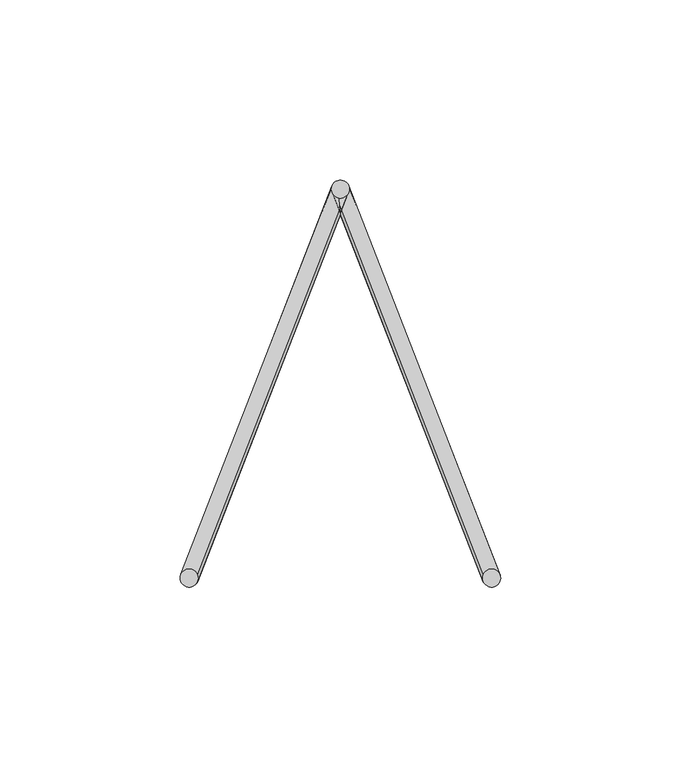
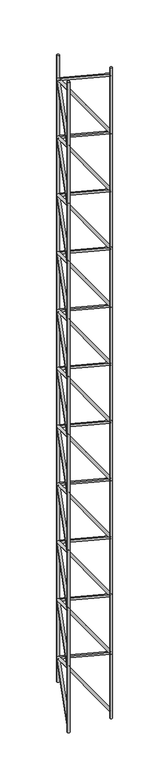
"""IFC4 building model written with IfcOpenShell, lengths in millimetres: proxy geometry, Pre-fab. (Vigota 1 - Pano 21)."""

from ifc_helpers import new_model, si_unit, point, frame, frame_2d, origin, origin_with_axes, origin_2d, place, context, project, spatial, circle_curve, trimmed, segment, composite_curve, outline, extrude, source, transform, mapped, element, save


def structural_framing_493db843(model_context):
    return source(origin(), model_context, "Body", "SweptSolid", [
        extrude(outline(composite_curve([segment(trimmed(circle_curve(origin_2d(), 2.5), [point((2.5, 0.0))], [point((-2.5, 0.0))], False, "CARTESIAN"), True, "CONTINUOUS"), segment(trimmed(circle_curve(origin_2d(), 2.5), [point((-2.5, 0.0))], [point((2.5, 0.0))], False, "CARTESIAN"), True, "CONTINUOUS")], self_intersect=False)), origin_with_axes(), (0.0, 0.0, 1.0), 1348.99893),
        extrude(outline(composite_curve([segment(trimmed(circle_curve(frame_2d((-42.0, 108.0)), 2.5), [point((-39.5, 108.0))], [point((-44.5, 108.0))], False, "CARTESIAN"), True, "CONTINUOUS"), segment(trimmed(circle_curve(frame_2d((-42.0, 108.0)), 2.5), [point((-44.5, 108.0))], [point((-39.5, 108.0))], False, "CARTESIAN"), True, "CONTINUOUS")], self_intersect=False)), frame((0.0, 0.0, 24.499465), z_axis=(0.0, 0.0, 1.0), x_axis=(1.0, 0.0, 0.0)), (0.0, 0.0, 1.0), 1300.0),
        extrude(outline(composite_curve([segment(trimmed(circle_curve(origin_2d(), 2.5), [point((2.5, 0.0))], [point((-2.5, 0.0))], False, "CARTESIAN"), True, "CONTINUOUS"), segment(trimmed(circle_curve(origin_2d(), 2.5), [point((-2.5, 0.0))], [point((2.5, 0.0))], False, "CARTESIAN"), True, "CONTINUOUS")], self_intersect=False)), frame((0.0, 0.0, 14.499465), z_axis=(-0.3218603428886276, 0.8276408817707567, 0.4598004898837537), x_axis=(0.8192319205108605, -3.936835275445103e-11, 0.5734623443750141)), (0.0, 0.0, 1.0), 130.491379),
        extrude(outline(composite_curve([segment(trimmed(circle_curve(origin_2d(), 2.5), [point((2.5, 0.0))], [point((-2.5, 0.0))], False, "CARTESIAN"), True, "CONTINUOUS"), segment(trimmed(circle_curve(origin_2d(), 2.5), [point((-2.5, 0.0))], [point((2.5, 0.0))], False, "CARTESIAN"), True, "CONTINUOUS")], self_intersect=False)), frame((-42.0, 108.0, 74.499465), z_axis=(0.3218603428886276, -0.8276408817707567, 0.4598004898837537), x_axis=(0.8192319205108605, -3.936835275445103e-11, -0.5734623443750141)), (0.0, 0.0, 1.0), 130.491379),
        extrude(outline(composite_curve([segment(trimmed(circle_curve(origin_2d(), 2.5), [point((2.5, 0.0))], [point((-2.5, 0.0))], False, "CARTESIAN"), True, "CONTINUOUS"), segment(trimmed(circle_curve(origin_2d(), 2.5), [point((-2.5, 0.0))], [point((2.5, 0.0))], False, "CARTESIAN"), True, "CONTINUOUS")], self_intersect=False)), frame((0.0, 0.0, 134.499465), z_axis=(-0.3218603428886276, 0.8276408817707567, 0.4598004898837537), x_axis=(0.8192319205108605, -3.936835275445103e-11, 0.5734623443750141)), (0.0, 0.0, 1.0), 130.491379),
        extrude(outline(composite_curve([segment(trimmed(circle_curve(origin_2d(), 2.5), [point((2.5, 0.0))], [point((-2.5, 0.0))], False, "CARTESIAN"), True, "CONTINUOUS"), segment(trimmed(circle_curve(origin_2d(), 2.5), [point((-2.5, 0.0))], [point((2.5, 0.0))], False, "CARTESIAN"), True, "CONTINUOUS")], self_intersect=False)), frame((-42.0, 108.0, 194.499465), z_axis=(0.3218603428886276, -0.8276408817707567, 0.4598004898837537), x_axis=(0.8192319205108605, -3.936835275445103e-11, -0.5734623443750141)), (0.0, 0.0, 1.0), 130.491379),
        extrude(outline(composite_curve([segment(trimmed(circle_curve(origin_2d(), 2.5), [point((2.5, 0.0))], [point((-2.5, 0.0))], False, "CARTESIAN"), True, "CONTINUOUS"), segment(trimmed(circle_curve(origin_2d(), 2.5), [point((-2.5, 0.0))], [point((2.5, 0.0))], False, "CARTESIAN"), True, "CONTINUOUS")], self_intersect=False)), frame((0.0, 0.0, 254.499465), z_axis=(-0.3218603428886276, 0.8276408817707567, 0.4598004898837537), x_axis=(0.8192319205108605, -3.936835275445103e-11, 0.5734623443750141)), (0.0, 0.0, 1.0), 130.491379),
        extrude(outline(composite_curve([segment(trimmed(circle_curve(origin_2d(), 2.5), [point((2.5, 0.0))], [point((-2.5, 0.0))], False, "CARTESIAN"), True, "CONTINUOUS"), segment(trimmed(circle_curve(origin_2d(), 2.5), [point((-2.5, 0.0))], [point((2.5, 0.0))], False, "CARTESIAN"), True, "CONTINUOUS")], self_intersect=False)), frame((-42.0, 108.0, 314.499465), z_axis=(0.3218603428886276, -0.8276408817707567, 0.4598004898837537), x_axis=(0.8192319205108605, -3.936835275445103e-11, -0.5734623443750141)), (0.0, 0.0, 1.0), 130.491379),
        extrude(outline(composite_curve([segment(trimmed(circle_curve(origin_2d(), 2.5), [point((2.5, 0.0))], [point((-2.5, 0.0))], False, "CARTESIAN"), True, "CONTINUOUS"), segment(trimmed(circle_curve(origin_2d(), 2.5), [point((-2.5, 0.0))], [point((2.5, 0.0))], False, "CARTESIAN"), True, "CONTINUOUS")], self_intersect=False)), frame((0.0, 0.0, 374.499465), z_axis=(-0.3218603428886276, 0.8276408817707567, 0.4598004898837537), x_axis=(0.8192319205108605, -3.936835275445103e-11, 0.5734623443750141)), (0.0, 0.0, 1.0), 130.491379),
        extrude(outline(composite_curve([segment(trimmed(circle_curve(origin_2d(), 2.5), [point((2.5, 0.0))], [point((-2.5, 0.0))], False, "CARTESIAN"), True, "CONTINUOUS"), segment(trimmed(circle_curve(origin_2d(), 2.5), [point((-2.5, 0.0))], [point((2.5, 0.0))], False, "CARTESIAN"), True, "CONTINUOUS")], self_intersect=False)), frame((-42.0, 108.0, 434.499465), z_axis=(0.3218603428886276, -0.8276408817707567, 0.4598004898837537), x_axis=(0.8192319205108605, -3.936835275445103e-11, -0.5734623443750141)), (0.0, 0.0, 1.0), 130.491379),
        extrude(outline(composite_curve([segment(trimmed(circle_curve(origin_2d(), 2.5), [point((2.5, 0.0))], [point((-2.5, 0.0))], False, "CARTESIAN"), True, "CONTINUOUS"), segment(trimmed(circle_curve(origin_2d(), 2.5), [point((-2.5, 0.0))], [point((2.5, 0.0))], False, "CARTESIAN"), True, "CONTINUOUS")], self_intersect=False)), frame((0.0, 0.0, 494.499465), z_axis=(-0.3218603428886276, 0.8276408817707567, 0.4598004898837537), x_axis=(0.8192319205108605, -3.936835275445103e-11, 0.5734623443750141)), (0.0, 0.0, 1.0), 130.491379),
        extrude(outline(composite_curve([segment(trimmed(circle_curve(origin_2d(), 2.5), [point((2.5, 0.0))], [point((-2.5, 0.0))], False, "CARTESIAN"), True, "CONTINUOUS"), segment(trimmed(circle_curve(origin_2d(), 2.5), [point((-2.5, 0.0))], [point((2.5, 0.0))], False, "CARTESIAN"), True, "CONTINUOUS")], self_intersect=False)), frame((-42.0, 108.0, 554.499465), z_axis=(0.3218603428886276, -0.8276408817707567, 0.4598004898837537), x_axis=(0.8192319205108605, -3.936835275445103e-11, -0.5734623443750141)), (0.0, 0.0, 1.0), 130.491379),
        extrude(outline(composite_curve([segment(trimmed(circle_curve(origin_2d(), 2.5), [point((2.5, 0.0))], [point((-2.5, 0.0))], False, "CARTESIAN"), True, "CONTINUOUS"), segment(trimmed(circle_curve(origin_2d(), 2.5), [point((-2.5, 0.0))], [point((2.5, 0.0))], False, "CARTESIAN"), True, "CONTINUOUS")], self_intersect=False)), frame((0.0, 0.0, 614.499465), z_axis=(-0.3218603428886276, 0.8276408817707567, 0.4598004898837537), x_axis=(0.8192319205108605, -3.936835275445103e-11, 0.5734623443750141)), (0.0, 0.0, 1.0), 130.491379),
        extrude(outline(composite_curve([segment(trimmed(circle_curve(origin_2d(), 2.5), [point((2.5, 0.0))], [point((-2.5, 0.0))], False, "CARTESIAN"), True, "CONTINUOUS"), segment(trimmed(circle_curve(origin_2d(), 2.5), [point((-2.5, 0.0))], [point((2.5, 0.0))], False, "CARTESIAN"), True, "CONTINUOUS")], self_intersect=False)), frame((-42.0, 108.0, 674.499465), z_axis=(0.3218603428886276, -0.8276408817707567, 0.4598004898837537), x_axis=(0.8192319205108605, -3.936835275445103e-11, -0.5734623443750141)), (0.0, 0.0, 1.0), 130.491379),
        extrude(outline(composite_curve([segment(trimmed(circle_curve(origin_2d(), 2.5), [point((2.5, 0.0))], [point((-2.5, 0.0))], False, "CARTESIAN"), True, "CONTINUOUS"), segment(trimmed(circle_curve(origin_2d(), 2.5), [point((-2.5, 0.0))], [point((2.5, 0.0))], False, "CARTESIAN"), True, "CONTINUOUS")], self_intersect=False)), frame((0.0, 0.0, 734.499465), z_axis=(-0.3218603428886276, 0.8276408817707567, 0.4598004898837537), x_axis=(0.8192319205108605, -3.936835275445103e-11, 0.5734623443750141)), (0.0, 0.0, 1.0), 130.491379),
        extrude(outline(composite_curve([segment(trimmed(circle_curve(origin_2d(), 2.5), [point((2.5, 0.0))], [point((-2.5, 0.0))], False, "CARTESIAN"), True, "CONTINUOUS"), segment(trimmed(circle_curve(origin_2d(), 2.5), [point((-2.5, 0.0))], [point((2.5, 0.0))], False, "CARTESIAN"), True, "CONTINUOUS")], self_intersect=False)), frame((-42.0, 108.0, 794.499465), z_axis=(0.3218603428886276, -0.8276408817707567, 0.4598004898837537), x_axis=(0.8192319205108605, -3.936835275445103e-11, -0.5734623443750141)), (0.0, 0.0, 1.0), 130.491379),
        extrude(outline(composite_curve([segment(trimmed(circle_curve(origin_2d(), 2.5), [point((2.5, 0.0))], [point((-2.5, 0.0))], False, "CARTESIAN"), True, "CONTINUOUS"), segment(trimmed(circle_curve(origin_2d(), 2.5), [point((-2.5, 0.0))], [point((2.5, 0.0))], False, "CARTESIAN"), True, "CONTINUOUS")], self_intersect=False)), frame((0.0, 0.0, 854.499465), z_axis=(-0.3218603428886276, 0.8276408817707567, 0.4598004898837537), x_axis=(0.8192319205108605, -3.936835275445103e-11, 0.5734623443750141)), (0.0, 0.0, 1.0), 130.491379),
        extrude(outline(composite_curve([segment(trimmed(circle_curve(origin_2d(), 2.5), [point((2.5, 0.0))], [point((-2.5, 0.0))], False, "CARTESIAN"), True, "CONTINUOUS"), segment(trimmed(circle_curve(origin_2d(), 2.5), [point((-2.5, 0.0))], [point((2.5, 0.0))], False, "CARTESIAN"), True, "CONTINUOUS")], self_intersect=False)), frame((-42.0, 108.0, 914.499465), z_axis=(0.3218603428886276, -0.8276408817707567, 0.4598004898837537), x_axis=(0.8192319205108605, -3.936835275445103e-11, -0.5734623443750141)), (0.0, 0.0, 1.0), 130.491379),
        extrude(outline(composite_curve([segment(trimmed(circle_curve(origin_2d(), 2.5), [point((2.5, 0.0))], [point((-2.5, 0.0))], False, "CARTESIAN"), True, "CONTINUOUS"), segment(trimmed(circle_curve(origin_2d(), 2.5), [point((-2.5, 0.0))], [point((2.5, 0.0))], False, "CARTESIAN"), True, "CONTINUOUS")], self_intersect=False)), frame((0.0, 0.0, 974.499465), z_axis=(-0.3218603428886276, 0.8276408817707567, 0.4598004898837537), x_axis=(0.8192319205108605, -3.936835275445103e-11, 0.5734623443750141)), (0.0, 0.0, 1.0), 130.491379),
        extrude(outline(composite_curve([segment(trimmed(circle_curve(origin_2d(), 2.5), [point((2.5, 0.0))], [point((-2.5, 0.0))], False, "CARTESIAN"), True, "CONTINUOUS"), segment(trimmed(circle_curve(origin_2d(), 2.5), [point((-2.5, 0.0))], [point((2.5, 0.0))], False, "CARTESIAN"), True, "CONTINUOUS")], self_intersect=False)), frame((-42.0, 108.0, 1034.499465), z_axis=(0.3218603428886276, -0.8276408817707567, 0.4598004898837537), x_axis=(0.8192319205108605, -3.936835275445103e-11, -0.5734623443750141)), (0.0, 0.0, 1.0), 130.491379),
        extrude(outline(composite_curve([segment(trimmed(circle_curve(origin_2d(), 2.5), [point((2.5, 0.0))], [point((-2.5, 0.0))], False, "CARTESIAN"), True, "CONTINUOUS"), segment(trimmed(circle_curve(origin_2d(), 2.5), [point((-2.5, 0.0))], [point((2.5, 0.0))], False, "CARTESIAN"), True, "CONTINUOUS")], self_intersect=False)), frame((0.0, 0.0, 1094.499465), z_axis=(-0.3218603428886276, 0.8276408817707567, 0.4598004898837537), x_axis=(0.8192319205108605, -3.936835275445103e-11, 0.5734623443750141)), (0.0, 0.0, 1.0), 130.491379),
        extrude(outline(composite_curve([segment(trimmed(circle_curve(origin_2d(), 2.5), [point((2.5, 0.0))], [point((-2.5, 0.0))], False, "CARTESIAN"), True, "CONTINUOUS"), segment(trimmed(circle_curve(origin_2d(), 2.5), [point((-2.5, 0.0))], [point((2.5, 0.0))], False, "CARTESIAN"), True, "CONTINUOUS")], self_intersect=False)), frame((-42.0, 108.0, 1154.499465), z_axis=(0.3218603428886276, -0.8276408817707567, 0.4598004898837537), x_axis=(0.8192319205108605, -3.936835275445103e-11, -0.5734623443750141)), (0.0, 0.0, 1.0), 130.491379),
        extrude(outline(composite_curve([segment(trimmed(circle_curve(origin_2d(), 2.5), [point((2.5, 0.0))], [point((-2.5, 0.0))], False, "CARTESIAN"), True, "CONTINUOUS"), segment(trimmed(circle_curve(origin_2d(), 2.5), [point((-2.5, 0.0))], [point((2.5, 0.0))], False, "CARTESIAN"), True, "CONTINUOUS")], self_intersect=False)), frame((0.0, 0.0, 1214.499465), z_axis=(-0.3218603428886276, 0.8276408817707567, 0.4598004898837537), x_axis=(0.8192319205108605, -3.936835275445103e-11, 0.5734623443750141)), (0.0, 0.0, 1.0), 130.491379),
        extrude(outline(composite_curve([segment(trimmed(circle_curve(origin_2d(), 2.5), [point((2.5, 0.0))], [point((-2.5, 0.0))], False, "CARTESIAN"), True, "CONTINUOUS"), segment(trimmed(circle_curve(origin_2d(), 2.5), [point((-2.5, 0.0))], [point((2.5, 0.0))], False, "CARTESIAN"), True, "CONTINUOUS")], self_intersect=False)), frame((-42.0, 108.0, 1274.499465), z_axis=(0.3218603428886276, -0.8276408817707567, 0.4598004898837537), x_axis=(0.8192319205108605, -3.936835275445103e-11, -0.5734623443750141)), (0.0, 0.0, 1.0), 130.491379),
        extrude(outline(composite_curve([segment(trimmed(circle_curve(frame_2d((-84.0, 0.0)), 2.5), [point((-81.5, 0.0))], [point((-86.5, 0.0))], False, "CARTESIAN"), True, "CONTINUOUS"), segment(trimmed(circle_curve(frame_2d((-84.0, 0.0)), 2.5), [point((-86.5, 0.0))], [point((-81.5, 0.0))], False, "CARTESIAN"), True, "CONTINUOUS")], self_intersect=False)), origin_with_axes(), (0.0, 0.0, 1.0), 1348.99893),
        extrude(outline(composite_curve([segment(trimmed(circle_curve(origin_2d(), 2.5), [point((2.5, 0.0))], [point((-2.5, 0.0))], False, "CARTESIAN"), True, "CONTINUOUS"), segment(trimmed(circle_curve(origin_2d(), 2.5), [point((-2.5, 0.0))], [point((2.5, 0.0))], False, "CARTESIAN"), True, "CONTINUOUS")], self_intersect=False)), frame((-84.0, 0.0, 14.499465), z_axis=(0.3218603428886276, 0.8276408817707567, 0.4598004898837537), x_axis=(0.8192319205108605, 3.936835275445103e-11, -0.5734623443750141)), (0.0, 0.0, 1.0), 130.491379),
        extrude(outline(composite_curve([segment(trimmed(circle_curve(origin_2d(), 2.5), [point((2.5, 0.0))], [point((-2.5, 0.0))], False, "CARTESIAN"), True, "CONTINUOUS"), segment(trimmed(circle_curve(origin_2d(), 2.5), [point((-2.5, 0.0))], [point((2.5, 0.0))], False, "CARTESIAN"), True, "CONTINUOUS")], self_intersect=False)), frame((-42.0, 108.0, 74.499465), z_axis=(-0.3218603428886276, -0.8276408817707567, 0.4598004898837537), x_axis=(0.8192319205108605, 3.936835275445103e-11, 0.5734623443750141)), (0.0, 0.0, 1.0), 130.491379),
        extrude(outline(composite_curve([segment(trimmed(circle_curve(origin_2d(), 2.5), [point((2.5, 0.0))], [point((-2.5, 0.0))], False, "CARTESIAN"), True, "CONTINUOUS"), segment(trimmed(circle_curve(origin_2d(), 2.5), [point((-2.5, 0.0))], [point((2.5, 0.0))], False, "CARTESIAN"), True, "CONTINUOUS")], self_intersect=False)), frame((-84.0, 0.0, 134.499465), z_axis=(0.3218603428886276, 0.8276408817707567, 0.4598004898837537), x_axis=(0.8192319205108605, 3.936835275445103e-11, -0.5734623443750141)), (0.0, 0.0, 1.0), 130.491379),
        extrude(outline(composite_curve([segment(trimmed(circle_curve(origin_2d(), 2.5), [point((2.5, 0.0))], [point((-2.5, 0.0))], False, "CARTESIAN"), True, "CONTINUOUS"), segment(trimmed(circle_curve(origin_2d(), 2.5), [point((-2.5, 0.0))], [point((2.5, 0.0))], False, "CARTESIAN"), True, "CONTINUOUS")], self_intersect=False)), frame((-42.0, 108.0, 194.499465), z_axis=(-0.3218603428886276, -0.8276408817707567, 0.4598004898837537), x_axis=(0.8192319205108605, 3.936835275445103e-11, 0.5734623443750141)), (0.0, 0.0, 1.0), 130.491379),
        extrude(outline(composite_curve([segment(trimmed(circle_curve(origin_2d(), 2.5), [point((2.5, 0.0))], [point((-2.5, 0.0))], False, "CARTESIAN"), True, "CONTINUOUS"), segment(trimmed(circle_curve(origin_2d(), 2.5), [point((-2.5, 0.0))], [point((2.5, 0.0))], False, "CARTESIAN"), True, "CONTINUOUS")], self_intersect=False)), frame((-84.0, 0.0, 254.499465), z_axis=(0.3218603428886276, 0.8276408817707567, 0.4598004898837537), x_axis=(0.8192319205108605, 3.936835275445103e-11, -0.5734623443750141)), (0.0, 0.0, 1.0), 130.491379),
        extrude(outline(composite_curve([segment(trimmed(circle_curve(origin_2d(), 2.5), [point((2.5, 0.0))], [point((-2.5, 0.0))], False, "CARTESIAN"), True, "CONTINUOUS"), segment(trimmed(circle_curve(origin_2d(), 2.5), [point((-2.5, 0.0))], [point((2.5, 0.0))], False, "CARTESIAN"), True, "CONTINUOUS")], self_intersect=False)), frame((-42.0, 108.0, 314.499465), z_axis=(-0.3218603428886276, -0.8276408817707567, 0.4598004898837537), x_axis=(0.8192319205108605, 3.936835275445103e-11, 0.5734623443750141)), (0.0, 0.0, 1.0), 130.491379),
        extrude(outline(composite_curve([segment(trimmed(circle_curve(origin_2d(), 2.5), [point((2.5, 0.0))], [point((-2.5, 0.0))], False, "CARTESIAN"), True, "CONTINUOUS"), segment(trimmed(circle_curve(origin_2d(), 2.5), [point((-2.5, 0.0))], [point((2.5, 0.0))], False, "CARTESIAN"), True, "CONTINUOUS")], self_intersect=False)), frame((-84.0, 0.0, 374.499465), z_axis=(0.3218603428886276, 0.8276408817707567, 0.4598004898837537), x_axis=(0.8192319205108605, 3.936835275445103e-11, -0.5734623443750141)), (0.0, 0.0, 1.0), 130.491379),
        extrude(outline(composite_curve([segment(trimmed(circle_curve(origin_2d(), 2.5), [point((2.5, 0.0))], [point((-2.5, 0.0))], False, "CARTESIAN"), True, "CONTINUOUS"), segment(trimmed(circle_curve(origin_2d(), 2.5), [point((-2.5, 0.0))], [point((2.5, 0.0))], False, "CARTESIAN"), True, "CONTINUOUS")], self_intersect=False)), frame((-42.0, 108.0, 434.499465), z_axis=(-0.3218603428886276, -0.8276408817707567, 0.4598004898837537), x_axis=(0.8192319205108605, 3.936835275445103e-11, 0.5734623443750141)), (0.0, 0.0, 1.0), 130.491379),
        extrude(outline(composite_curve([segment(trimmed(circle_curve(origin_2d(), 2.5), [point((2.5, 0.0))], [point((-2.5, 0.0))], False, "CARTESIAN"), True, "CONTINUOUS"), segment(trimmed(circle_curve(origin_2d(), 2.5), [point((-2.5, 0.0))], [point((2.5, 0.0))], False, "CARTESIAN"), True, "CONTINUOUS")], self_intersect=False)), frame((-84.0, 0.0, 494.499465), z_axis=(0.3218603428886276, 0.8276408817707567, 0.4598004898837537), x_axis=(0.8192319205108605, 3.936835275445103e-11, -0.5734623443750141)), (0.0, 0.0, 1.0), 130.491379),
        extrude(outline(composite_curve([segment(trimmed(circle_curve(origin_2d(), 2.5), [point((2.5, 0.0))], [point((-2.5, 0.0))], False, "CARTESIAN"), True, "CONTINUOUS"), segment(trimmed(circle_curve(origin_2d(), 2.5), [point((-2.5, 0.0))], [point((2.5, 0.0))], False, "CARTESIAN"), True, "CONTINUOUS")], self_intersect=False)), frame((-42.0, 108.0, 554.499465), z_axis=(-0.3218603428886276, -0.8276408817707567, 0.4598004898837537), x_axis=(0.8192319205108605, 3.936835275445103e-11, 0.5734623443750141)), (0.0, 0.0, 1.0), 130.491379),
        extrude(outline(composite_curve([segment(trimmed(circle_curve(origin_2d(), 2.5), [point((2.5, 0.0))], [point((-2.5, 0.0))], False, "CARTESIAN"), True, "CONTINUOUS"), segment(trimmed(circle_curve(origin_2d(), 2.5), [point((-2.5, 0.0))], [point((2.5, 0.0))], False, "CARTESIAN"), True, "CONTINUOUS")], self_intersect=False)), frame((-84.0, 0.0, 614.499465), z_axis=(0.3218603428886276, 0.8276408817707567, 0.4598004898837537), x_axis=(0.8192319205108605, 3.936835275445103e-11, -0.5734623443750141)), (0.0, 0.0, 1.0), 130.491379),
        extrude(outline(composite_curve([segment(trimmed(circle_curve(origin_2d(), 2.5), [point((2.5, 0.0))], [point((-2.5, 0.0))], False, "CARTESIAN"), True, "CONTINUOUS"), segment(trimmed(circle_curve(origin_2d(), 2.5), [point((-2.5, 0.0))], [point((2.5, 0.0))], False, "CARTESIAN"), True, "CONTINUOUS")], self_intersect=False)), frame((-42.0, 108.0, 674.499465), z_axis=(-0.3218603428886276, -0.8276408817707567, 0.4598004898837537), x_axis=(0.8192319205108605, 3.936835275445103e-11, 0.5734623443750141)), (0.0, 0.0, 1.0), 130.491379),
        extrude(outline(composite_curve([segment(trimmed(circle_curve(origin_2d(), 2.5), [point((2.5, 0.0))], [point((-2.5, 0.0))], False, "CARTESIAN"), True, "CONTINUOUS"), segment(trimmed(circle_curve(origin_2d(), 2.5), [point((-2.5, 0.0))], [point((2.5, 0.0))], False, "CARTESIAN"), True, "CONTINUOUS")], self_intersect=False)), frame((-84.0, 0.0, 734.499465), z_axis=(0.3218603428886276, 0.8276408817707567, 0.4598004898837537), x_axis=(0.8192319205108605, 3.936835275445103e-11, -0.5734623443750141)), (0.0, 0.0, 1.0), 130.491379),
        extrude(outline(composite_curve([segment(trimmed(circle_curve(origin_2d(), 2.5), [point((2.5, 0.0))], [point((-2.5, 0.0))], False, "CARTESIAN"), True, "CONTINUOUS"), segment(trimmed(circle_curve(origin_2d(), 2.5), [point((-2.5, 0.0))], [point((2.5, 0.0))], False, "CARTESIAN"), True, "CONTINUOUS")], self_intersect=False)), frame((-42.0, 108.0, 794.499465), z_axis=(-0.3218603428886276, -0.8276408817707567, 0.4598004898837537), x_axis=(0.8192319205108605, 3.936835275445103e-11, 0.5734623443750141)), (0.0, 0.0, 1.0), 130.491379),
        extrude(outline(composite_curve([segment(trimmed(circle_curve(origin_2d(), 2.5), [point((2.5, 0.0))], [point((-2.5, 0.0))], False, "CARTESIAN"), True, "CONTINUOUS"), segment(trimmed(circle_curve(origin_2d(), 2.5), [point((-2.5, 0.0))], [point((2.5, 0.0))], False, "CARTESIAN"), True, "CONTINUOUS")], self_intersect=False)), frame((-84.0, 0.0, 854.499465), z_axis=(0.3218603428886276, 0.8276408817707567, 0.4598004898837537), x_axis=(0.8192319205108605, 3.936835275445103e-11, -0.5734623443750141)), (0.0, 0.0, 1.0), 130.491379),
        extrude(outline(composite_curve([segment(trimmed(circle_curve(origin_2d(), 2.5), [point((2.5, 0.0))], [point((-2.5, 0.0))], False, "CARTESIAN"), True, "CONTINUOUS"), segment(trimmed(circle_curve(origin_2d(), 2.5), [point((-2.5, 0.0))], [point((2.5, 0.0))], False, "CARTESIAN"), True, "CONTINUOUS")], self_intersect=False)), frame((-42.0, 108.0, 914.499465), z_axis=(-0.3218603428886276, -0.8276408817707567, 0.4598004898837537), x_axis=(0.8192319205108605, 3.936835275445103e-11, 0.5734623443750141)), (0.0, 0.0, 1.0), 130.491379),
        extrude(outline(composite_curve([segment(trimmed(circle_curve(origin_2d(), 2.5), [point((2.5, 0.0))], [point((-2.5, 0.0))], False, "CARTESIAN"), True, "CONTINUOUS"), segment(trimmed(circle_curve(origin_2d(), 2.5), [point((-2.5, 0.0))], [point((2.5, 0.0))], False, "CARTESIAN"), True, "CONTINUOUS")], self_intersect=False)), frame((-84.0, 0.0, 974.499465), z_axis=(0.3218603428886276, 0.8276408817707567, 0.4598004898837537), x_axis=(0.8192319205108605, 3.936835275445103e-11, -0.5734623443750141)), (0.0, 0.0, 1.0), 130.491379),
        extrude(outline(composite_curve([segment(trimmed(circle_curve(origin_2d(), 2.5), [point((2.5, 0.0))], [point((-2.5, 0.0))], False, "CARTESIAN"), True, "CONTINUOUS"), segment(trimmed(circle_curve(origin_2d(), 2.5), [point((-2.5, 0.0))], [point((2.5, 0.0))], False, "CARTESIAN"), True, "CONTINUOUS")], self_intersect=False)), frame((-42.0, 108.0, 1034.499465), z_axis=(-0.3218603428886276, -0.8276408817707567, 0.4598004898837537), x_axis=(0.8192319205108605, 3.936835275445103e-11, 0.5734623443750141)), (0.0, 0.0, 1.0), 130.491379),
        extrude(outline(composite_curve([segment(trimmed(circle_curve(origin_2d(), 2.5), [point((2.5, 0.0))], [point((-2.5, 0.0))], False, "CARTESIAN"), True, "CONTINUOUS"), segment(trimmed(circle_curve(origin_2d(), 2.5), [point((-2.5, 0.0))], [point((2.5, 0.0))], False, "CARTESIAN"), True, "CONTINUOUS")], self_intersect=False)), frame((-84.0, 0.0, 1094.499465), z_axis=(0.3218603428886276, 0.8276408817707567, 0.4598004898837537), x_axis=(0.8192319205108605, 3.936835275445103e-11, -0.5734623443750141)), (0.0, 0.0, 1.0), 130.491379),
        extrude(outline(composite_curve([segment(trimmed(circle_curve(origin_2d(), 2.5), [point((2.5, 0.0))], [point((-2.5, 0.0))], False, "CARTESIAN"), True, "CONTINUOUS"), segment(trimmed(circle_curve(origin_2d(), 2.5), [point((-2.5, 0.0))], [point((2.5, 0.0))], False, "CARTESIAN"), True, "CONTINUOUS")], self_intersect=False)), frame((-42.0, 108.0, 1154.499465), z_axis=(-0.3218603428886276, -0.8276408817707567, 0.4598004898837537), x_axis=(0.8192319205108605, 3.936835275445103e-11, 0.5734623443750141)), (0.0, 0.0, 1.0), 130.491379),
        extrude(outline(composite_curve([segment(trimmed(circle_curve(origin_2d(), 2.5), [point((2.5, 0.0))], [point((-2.5, 0.0))], False, "CARTESIAN"), True, "CONTINUOUS"), segment(trimmed(circle_curve(origin_2d(), 2.5), [point((-2.5, 0.0))], [point((2.5, 0.0))], False, "CARTESIAN"), True, "CONTINUOUS")], self_intersect=False)), frame((-84.0, 0.0, 1214.499465), z_axis=(0.3218603428886276, 0.8276408817707567, 0.4598004898837537), x_axis=(0.8192319205108605, 3.936835275445103e-11, -0.5734623443750141)), (0.0, 0.0, 1.0), 130.491379),
        extrude(outline(composite_curve([segment(trimmed(circle_curve(origin_2d(), 2.5), [point((2.5, 0.0))], [point((-2.5, 0.0))], False, "CARTESIAN"), True, "CONTINUOUS"), segment(trimmed(circle_curve(origin_2d(), 2.5), [point((-2.5, 0.0))], [point((2.5, 0.0))], False, "CARTESIAN"), True, "CONTINUOUS")], self_intersect=False)), frame((-42.0, 108.0, 1274.499465), z_axis=(-0.3218603428886276, -0.8276408817707567, 0.4598004898837537), x_axis=(0.8192319205108605, 3.936835275445103e-11, 0.5734623443750141)), (0.0, 0.0, 1.0), 130.491379),
    ])


if __name__ == "__main__":
    model = new_model("IFC4")
    model_context = context("Model", 3, world=origin())
    ifc_project = project(units=[si_unit("LENGTHUNIT", "METRE", prefix="MILLI")], contexts=[model_context])
    site = spatial("IfcSite", under=ifc_project)
    building = spatial("IfcBuilding", under=site)
    placement = place(None, origin())
    structural_framing_shape = structural_framing_493db843(model_context)
    element("IfcBuildingElementProxy", 1, Name="Pre-fab. (Vigota 1 - Pano 21)", ObjectType="Pre-fab. (Vigota 1 - Pano 21)", at=placement, inside=building, context=model_context, shape_type="MappedRepresentation", body=[
        mapped(structural_framing_shape, transform((0.0, 0.0, 0.0), x_axis=(1.0, 0.0, 0.0), y_axis=(0.0, 1.0, 0.0), z_axis=(0.0, 0.0, 1.0))),
    ])
    save(model, "model.ifc")

# Revit data of these elements
# Element 1 (IfcBuildingElementProxy, "Pre-fab. (Vigota 1 - Pano 21)")
#   Materials on its faces: "Aço"
# Materials
#   "Aço": class "Metal", colour RGB 120 120 120, transparency 0, Description = "Aço estrutural A36 grau, ASTM B, acabamento laminado", Cost = 0
